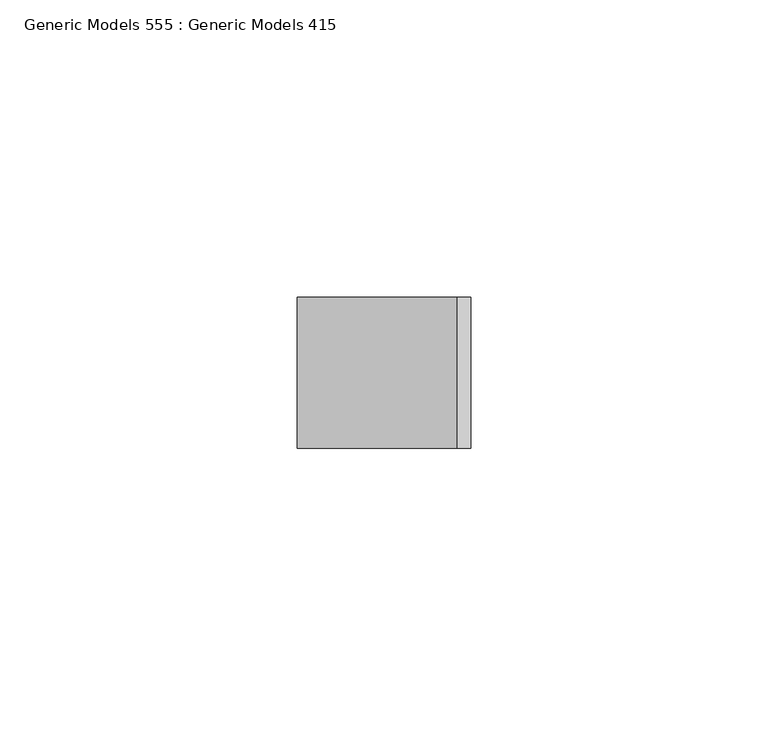
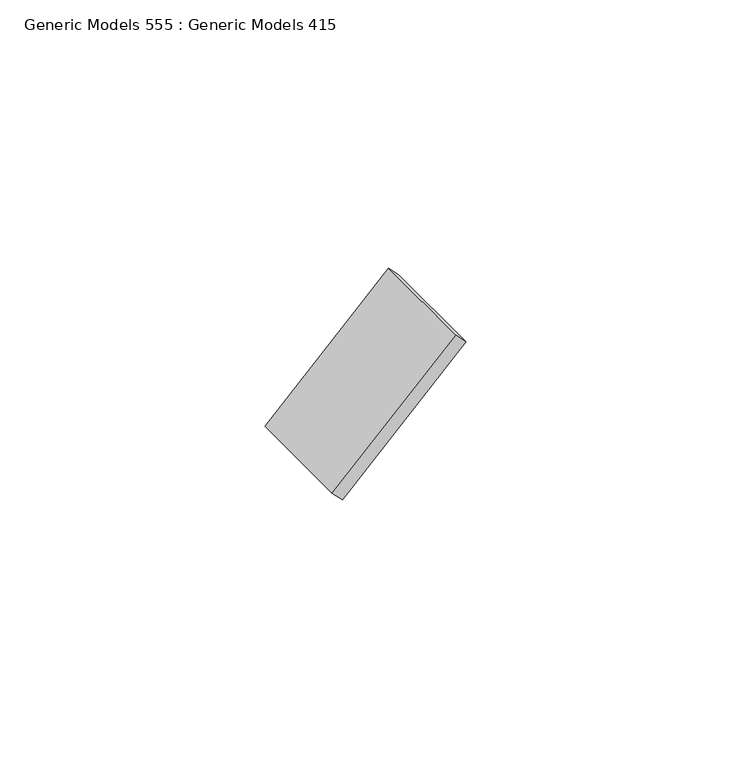
"""IFC4 building model written with IfcOpenShell, lengths in millimetres: proxy geometry, Generic Models 555 : Generic Models 415."""

from ifc_helpers import new_model, si_unit, frame, origin, place, context, project, spatial, polyline, outline, extrude, source, transform, mapped, element, save


def generic_models_555_generic_models_415_76ad5be0(model_context):
    return source(origin(), model_context, "Body", "SweptSolid", [
        extrude(outline(polyline([(0.0, -3.175), (0.0, 0.0), (25.4, 0.0), (25.4, -3.175), (0.0, -3.175)])), frame((7848.0411784, 4501.3863946, 124559.3849742), z_axis=(0.7071067811867181, 0.0, 0.707106781186377), x_axis=(0.0, -1.0, 0.0)), (0.0, 0.0, 1.0), 38.1),
    ])


if __name__ == "__main__":
    model = new_model("IFC4")
    model_context = context("Model", 3, world=origin())
    ifc_project = project(units=[si_unit("LENGTHUNIT", "METRE", prefix="MILLI")], contexts=[model_context])
    site = spatial("IfcSite", under=ifc_project)
    building = spatial("IfcBuilding", under=site)
    placement = place(None, origin())
    generic_models_555_generic_models_415_shape = generic_models_555_generic_models_415_76ad5be0(model_context)
    element("IfcBuildingElementProxy", 1, Name="Generic Models 555 : Generic Models 415", ObjectType="Generic Models 555 : Generic Models 415", at=placement, inside=building, context=model_context, shape_type="MappedRepresentation", body=[
        mapped(generic_models_555_generic_models_415_shape, transform((0.0, 0.0, 0.0), x_axis=(1.0, 0.0, 0.0), y_axis=(0.0, 1.0, 0.0), z_axis=(0.0, 0.0, 1.0))),
    ])
    save(model, "model.ifc")

# Revit data of these elements
# Element 1 (IfcBuildingElementProxy, "Generic Models 555 : Generic Models 415")
#   Materials on its faces: "_WELDED STEEL TABS FOR LOUVER ATTACHMENT"
# Materials
#   "_WELDED STEEL TABS FOR LOUVER ATTACHMENT": class "Metal", colour RGB 199 199 199, transparency 0, Description = "Structural steel 50ksi", Cost = 0
